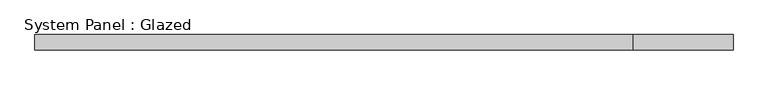
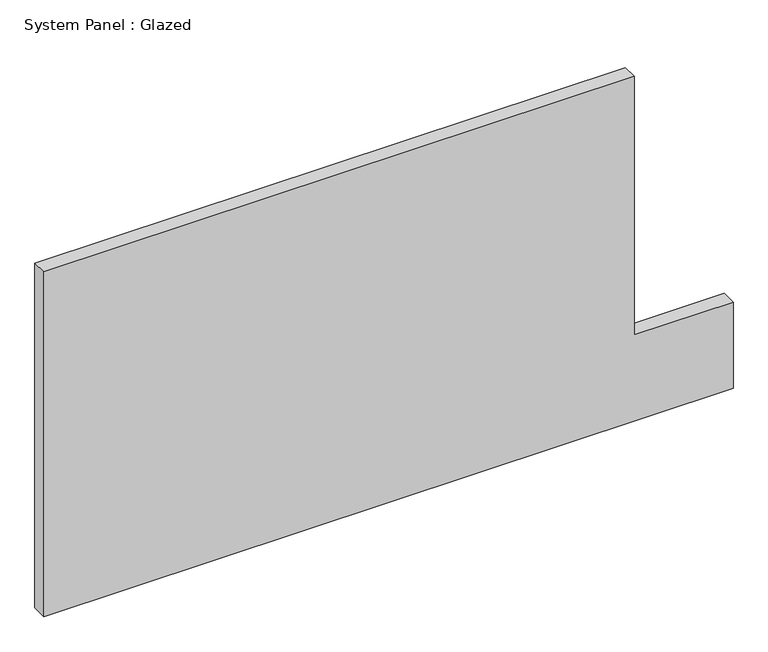
"""IFC4 building model written with IfcOpenShell, lengths in millimetres: plate geometry, System Panel : Glazed."""

from ifc_helpers import new_model, si_unit, frame, origin, place, context, project, spatial, polyline, outline, extrude, source, transform, mapped, element, save


def system_panel_glazed_d863b2e2(model_context):
    return source(origin(), model_context, "Body", "SweptSolid", [
        extrude(outline(polyline([(0.0, -576.624914), (0.0, 576.624914), (152.4, 576.624914), (152.4, 410.8942588), (609.6, 410.8942588), (609.6, -576.624914), (0.0, -576.624914)])), frame((0.0, 19.05, 0.0), z_axis=(0.0, 1.0, 0.0), x_axis=(0.0, 0.0, 1.0)), (0.0, 0.0, 1.0), 25.4),
    ])


if __name__ == "__main__":
    model = new_model("IFC4")
    model_context = context("Model", 3, world=origin())
    ifc_project = project(units=[si_unit("LENGTHUNIT", "METRE", prefix="MILLI")], contexts=[model_context])
    site = spatial("IfcSite", under=ifc_project)
    building = spatial("IfcBuilding", under=site)
    placement = place(None, origin())
    system_panel_glazed_shape = system_panel_glazed_d863b2e2(model_context)
    element("IfcPlate", 1, ObjectType="System Panel : Glazed", at=placement, inside=building, context=model_context, shape_type="MappedRepresentation", body=[
        mapped(system_panel_glazed_shape, transform((0.0, 0.0, 0.0), x_axis=(1.0, 0.0, 0.0), y_axis=(0.0, 1.0, 0.0), z_axis=(0.0, 0.0, 1.0))),
    ])
    save(model, "model.ifc")

# Revit data of these elements
# Element 1 (IfcPlate, "System Panel : Glazed")
#   Materials on its faces: "Glass"
# Materials
#   "Glass": class "Glass", colour RGB 0 128 192, transparency 0.75
